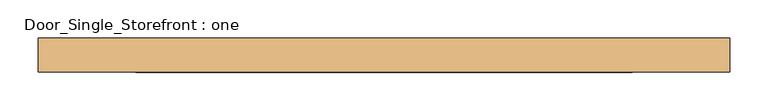
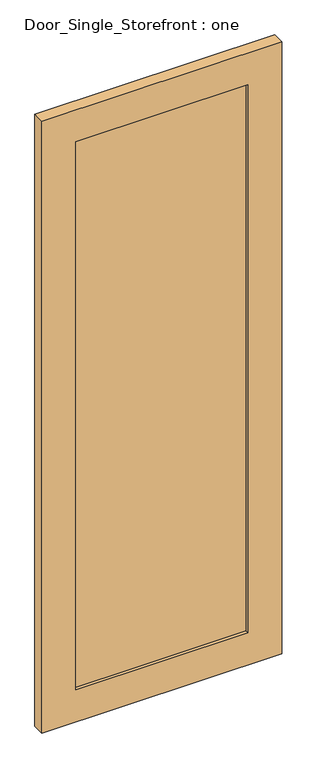
"""IFC4 building model written with IfcOpenShell, lengths in millimetres: door geometry, Door_Single_Storefront : one."""

import ifcopenshell
import ifcopenshell.guid

model = None  # the IFC model being written
_history = None  # IfcOwnerHistory: only IFC2X3 demands one
_inside = {}  # id of a spatial element -> (the spatial element, [elements in it])
_under = {}  # id of a project, library or spatial element -> (it, [spatial elements below it])
_declared = {}  # id of a project -> (the project, [libraries it declares])
_typed = {}  # id of a type object -> (the type object, [elements of that type])
_made_of = {}  # id of a material, layer set ... -> (it, [elements and type objects made of it])


def new_model(schema):
    """Start an empty IFC model of exactly this schema.

    Asked for "IFC4X3", IfcOpenShell would pick the latest addendum, in which some entities
    have other attributes; the version numbers below select the first issue.
    IFC2X3 requires an IfcOwnerHistory on every rooted entity: one is made here for all.
    """
    global model, _history
    if schema == "IFC4X3":
        model = ifcopenshell.file(schema_version=(4, 3, 0, 0))
    else:
        model = ifcopenshell.file(schema=schema)
    _inside.clear()
    _under.clear()
    _declared.clear()
    _typed.clear()
    _made_of.clear()
    _history = None
    if model.schema == "IFC2X3":
        org = make("IfcOrganization", Name="unknown")
        user = make(
            "IfcPersonAndOrganization",
            ThePerson=make("IfcPerson", FamilyName="unknown"),
            TheOrganization=org,
        )
        app = make(
            "IfcApplication",
            ApplicationDeveloper=org,
            Version="unknown",
            ApplicationFullName="unknown",
            ApplicationIdentifier="unknown",
        )
        _history = make(
            "IfcOwnerHistory",
            OwningUser=user,
            OwningApplication=app,
            ChangeAction="ADDED",
            CreationDate=0,
        )
    return model


def make(cls, **values):
    """One entity of the class cls with the attributes given. An attribute that is None is left unset."""
    return model.create_entity(
        cls, **{name: value for name, value in values.items() if value is not None}
    )


def rooted(cls, **values):
    """An entity with a GlobalId (a new one), such as an element, a storey or a relation."""
    return make(cls, GlobalId=ifcopenshell.guid.new(), OwnerHistory=_history, **values)


def si_unit(unit_type, name, prefix=None):
    """IfcSIUnit, for example si_unit("LENGTHUNIT", "METRE", prefix="MILLI")."""
    return make("IfcSIUnit", UnitType=unit_type, Prefix=prefix, Name=name)


def assignment(units):
    """IfcUnitAssignment: the units of a project."""
    return None if units is None else make("IfcUnitAssignment", Units=units)


def point(xyz):
    """IfcCartesianPoint."""
    return None if xyz is None else make("IfcCartesianPoint", Coordinates=xyz)


def direction(xyz):
    """IfcDirection."""
    return None if xyz is None else make("IfcDirection", DirectionRatios=xyz)


def frame(location, z_axis=None, x_axis=None):
    """IfcAxis2Placement3D, a coordinate frame: its origin and axes. An axis left out is left unset."""
    return make(
        "IfcAxis2Placement3D",
        Location=point(location),
        Axis=direction(z_axis),
        RefDirection=direction(x_axis),
    )


def origin():
    """The frame at (0, 0, 0) with its axes left unset."""
    return frame((0.0, 0.0, 0.0))


def place(relative_to, where):
    """IfcLocalPlacement: puts the frame where relative to a parent placement (None: the world)."""
    return make(
        "IfcLocalPlacement", PlacementRelTo=relative_to, RelativePlacement=where
    )


def context(
    kind, dimensions, precision=None, world=None, true_north=None, identifier=None
):
    """IfcGeometricRepresentationContext, for example the 3D "Model" context."""
    return make(
        "IfcGeometricRepresentationContext",
        ContextIdentifier=identifier,
        ContextType=kind,
        CoordinateSpaceDimension=dimensions,
        Precision=precision,
        WorldCoordinateSystem=world,
        TrueNorth=true_north,
    )


def project(units=None, contexts=None):
    """IfcProject with its units and contexts."""
    return rooted(
        "IfcProject",
        Name="project",
        RepresentationContexts=contexts,
        UnitsInContext=assignment(units),
    )


def spatial(cls, under=None, at=None, **own):
    """A site, building, storey or space (cls), placed at a placement, below another one or the project."""
    s = rooted(cls, ObjectPlacement=at, **own)
    if under is not None:
        _under.setdefault(under.id(), (under, []))[1].append(s)
    return s


def polyline(points):
    """IfcPolyline through the points."""
    return make("IfcPolyline", Points=[point(p) for p in points])


def outline(outer, holes=None, kind="AREA"):
    """IfcArbitraryClosedProfileDef: a profile drawn as a closed curve; with holes, ...WithVoids."""
    if holes is None:
        return make("IfcArbitraryClosedProfileDef", ProfileType=kind, OuterCurve=outer)
    return make(
        "IfcArbitraryProfileDefWithVoids",
        ProfileType=kind,
        OuterCurve=outer,
        InnerCurves=holes,
    )


def extrude(swept, where, along, depth):
    """IfcExtrudedAreaSolid: the profile swept, set in the frame where, extruded along a direction by depth."""
    return make(
        "IfcExtrudedAreaSolid",
        SweptArea=swept,
        Position=where,
        ExtrudedDirection=direction(along),
        Depth=depth,
    )


def shape(context_of_items, identifier, shape_type, items):
    """IfcShapeRepresentation: the items that make up one representation, for example the "Body"."""
    return make(
        "IfcShapeRepresentation",
        ContextOfItems=context_of_items,
        RepresentationIdentifier=identifier,
        RepresentationType=shape_type,
        Items=items,
    )


def source(mapping_origin, context_of_items, identifier, shape_type, items):
    """IfcRepresentationMap: a shape defined once, which mapped items show again and again."""
    return make(
        "IfcRepresentationMap",
        MappingOrigin=mapping_origin,
        MappedRepresentation=shape(context_of_items, identifier, shape_type, items),
    )


def transform(
    local_origin,
    x_axis=None,
    y_axis=None,
    z_axis=None,
    scale=None,
    scale2=None,
    scale3=None,
    uniform=True,
):
    """IfcCartesianTransformationOperator3D, or its non-uniform kind. x_axis, y_axis, z_axis: its Axis1, 2, 3."""
    if uniform:
        return make(
            "IfcCartesianTransformationOperator3D",
            Axis1=direction(x_axis),
            Axis2=direction(y_axis),
            LocalOrigin=point(local_origin),
            Scale=scale,
            Axis3=direction(z_axis),
        )
    return make(
        "IfcCartesianTransformationOperator3DnonUniform",
        Axis1=direction(x_axis),
        Axis2=direction(y_axis),
        LocalOrigin=point(local_origin),
        Scale=scale,
        Axis3=direction(z_axis),
        Scale2=scale2,
        Scale3=scale3,
    )


def mapped(mapping_source, mapping_target):
    """IfcMappedItem: shows the shape of a source again, moved by a transform."""
    return make(
        "IfcMappedItem", MappingSource=mapping_source, MappingTarget=mapping_target
    )


def made_of(thing, what):
    """Note that an element or type object is made of a material, layer set ...; save() writes the relation."""
    if what is not None:
        _made_of.setdefault(what.id(), (what, []))[1].append(thing)
    return thing


def element(
    cls,
    number,
    at=None,
    inside=None,
    cuts=None,
    type_object=None,
    material=None,
    context=None,
    identifier="Body",
    shape_type=None,
    held_by="IfcProductDefinitionShape",
    body=None,
    shapes=None,
    **own,
):
    """One element of the class cls, such as IfcWall. Its Tag is "e" and its number.

    at: its placement. inside: the storey or other place that contains it. cuts: it is an
    opening in that element (IfcRelVoidsElement). A single representation is given by context,
    identifier, shape_type and body (its items); several are given by shapes. held_by: the class
    of the entity that holds the representations. save() writes the other relations.
    """
    e = rooted(cls, Tag="e%d" % number, ObjectPlacement=at, **own)
    if body is not None:
        shapes = [shape(context, identifier, shape_type, body)]
    if shapes is not None:
        e.Representation = make(held_by, Representations=shapes)
    if inside is not None:
        _inside.setdefault(inside.id(), (inside, []))[1].append(e)
    if cuts is not None:
        rooted(
            "IfcRelVoidsElement", RelatingBuildingElement=cuts, RelatedOpeningElement=e
        )
    if type_object is not None:
        _typed.setdefault(type_object.id(), (type_object, []))[1].append(e)
    return made_of(e, material)


def aggregate(whole, parts):
    """IfcRelAggregates: a whole, such as a stair, and the parts it consists of."""
    return rooted("IfcRelAggregates", RelatingObject=whole, RelatedObjects=parts)


def save(model, path):
    """Write the relations noted so far, then the file.

    IfcRelAggregates (storeys below a building ...), IfcRelContainedInSpatialStructure (elements
    in a storey), IfcRelDefinesByType, IfcRelAssociatesMaterial and IfcRelDeclares: one each for
    every whole, place, type object, material and project.
    """
    for whole, parts in _under.values():
        aggregate(whole, parts)
    for where, things in _inside.values():
        rooted(
            "IfcRelContainedInSpatialStructure",
            RelatedElements=things,
            RelatingStructure=where,
        )
    for kind, things in _typed.values():
        rooted("IfcRelDefinesByType", RelatedObjects=things, RelatingType=kind)
    for what, things in _made_of.values():
        rooted("IfcRelAssociatesMaterial", RelatedObjects=things, RelatingMaterial=what)
    for by, libraries in _declared.values():
        rooted("IfcRelDeclares", RelatingContext=by, RelatedDefinitions=libraries)
    model.write(path)


def door_single_storefront_one_eb725c03(model_context):
    return source(origin(), model_context, "Body", "SweptSolid", [
        extrude(outline(polyline([(323.85, -6.35), (-323.85, -6.35), (-323.85, 12.7), (323.85, 12.7), (323.85, -6.35)])), frame((0.0, 0.0, 127.0), z_axis=(0.0, 0.0, 1.0), x_axis=(1.0, 0.0, 0.0)), (0.0, 0.0, 1.0), 2178.05),
        extrude(outline(polyline([(2432.05, -450.85), (0.0, -450.85), (0.0, 450.85), (2432.05, 450.85), (2432.05, -450.85)]), holes=[polyline([(127.0, 323.85), (127.0, -323.85), (2305.05, -323.85), (2305.05, 323.85), (127.0, 323.85)])]), frame((0.0, -19.05, 0.0), z_axis=(0.0, 1.0, 0.0), x_axis=(0.0, 0.0, 1.0)), (0.0, 0.0, 1.0), 44.45),
    ])


if __name__ == "__main__":
    model = new_model("IFC4")
    model_context = context("Model", 3, world=origin())
    ifc_project = project(units=[si_unit("LENGTHUNIT", "METRE", prefix="MILLI")], contexts=[model_context])
    site = spatial("IfcSite", under=ifc_project)
    building = spatial("IfcBuilding", under=site)
    placement = place(None, origin())
    door_single_storefront_one_shape = door_single_storefront_one_eb725c03(model_context)
    element("IfcDoor", 1, ObjectType="Door_Single_Storefront : one", at=placement, inside=building, context=model_context, shape_type="MappedRepresentation", body=[
        mapped(door_single_storefront_one_shape, transform((0.0, 0.0, 0.0), x_axis=(1.0, 0.0, 0.0), y_axis=(0.0, 1.0, 0.0), z_axis=(0.0, 0.0, 1.0))),
    ])
    save(model, "model.ifc")

# Revit data of these elements
# Type "Door_Single_Storefront : one"
#   Type Mark = "27"
#   Analytic Construction = "<None>"
#   Stile_Width = 0' - 5"
#   Door_Thickness = 0' - 1 3/4"
#   Door_Offset = 0' - 1"
#   Glass_Material = SAFETY GLAZING
#   Frame_Material = INTERIOR GRADE ALUMINUM STOREFRONT W/ SAFETY GLAZING
#   Function = (empty or 0)
# Element 1 (IfcDoor, "Door_Single_Storefront : one")
#   Materials on its faces: "INTERIOR GRADE ALUMINUM STOREFRONT W/ SAFETY GLAZING", "SAFETY GLAZING"
# Materials
#   "SAFETY GLAZING": class "Glass", colour RGB 142 168 196, transparency 0.75, Description = "Soda Lime Glass", Cost = 0
#   "INTERIOR GRADE ALUMINUM STOREFRONT W/ SAFETY GLAZING": class "Metal", colour RGB 226 226 226, transparency 0, Description = "Aluminum 6061", Cost = 0
